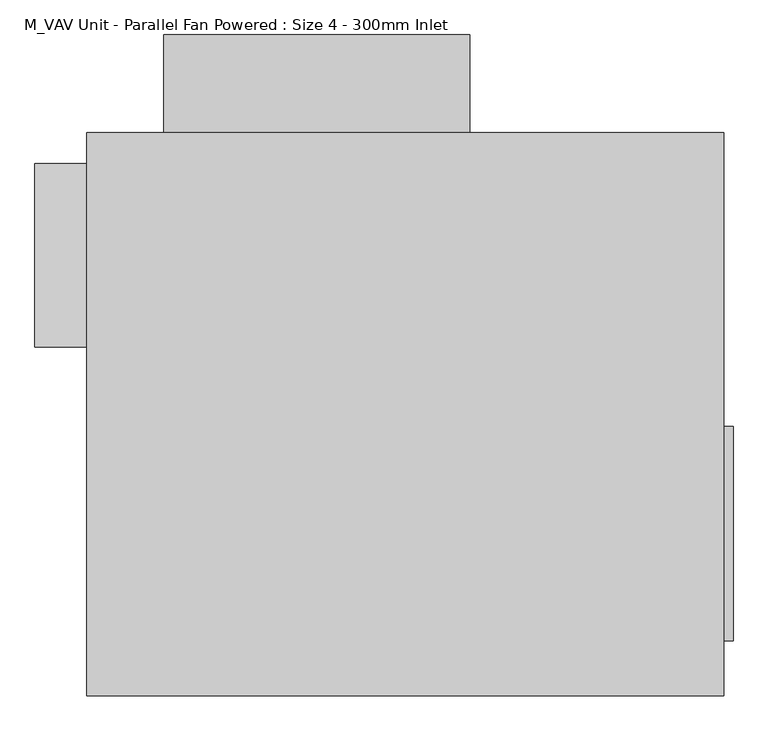
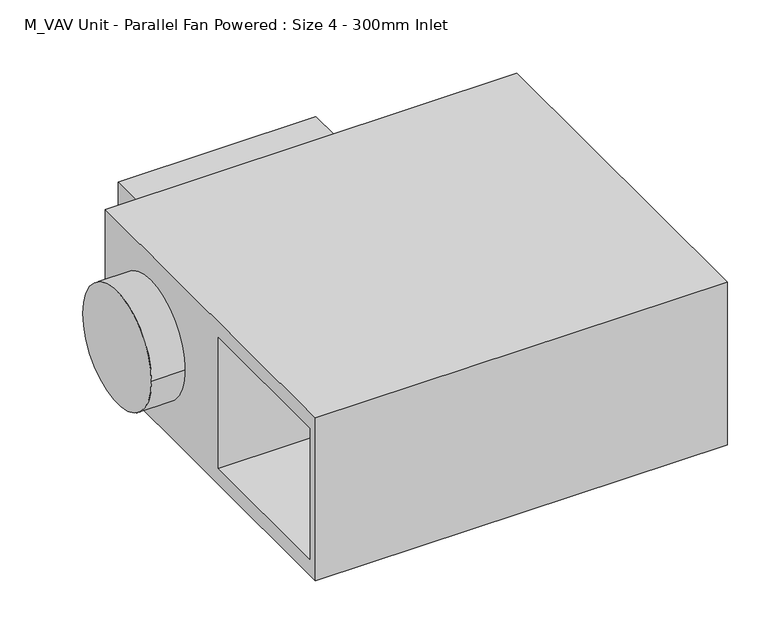
"""IFC4 building model written with IfcOpenShell, lengths in millimetres: proxy geometry, M_VAV Unit - Parallel Fan Powered : Size 4 - 300mm Inlet."""

import ifcopenshell
import ifcopenshell.guid

model = None  # the IFC model being written
_history = None  # IfcOwnerHistory: only IFC2X3 demands one
_inside = {}  # id of a spatial element -> (the spatial element, [elements in it])
_under = {}  # id of a project, library or spatial element -> (it, [spatial elements below it])
_declared = {}  # id of a project -> (the project, [libraries it declares])
_typed = {}  # id of a type object -> (the type object, [elements of that type])
_made_of = {}  # id of a material, layer set ... -> (it, [elements and type objects made of it])


def new_model(schema):
    """Start an empty IFC model of exactly this schema.

    Asked for "IFC4X3", IfcOpenShell would pick the latest addendum, in which some entities
    have other attributes; the version numbers below select the first issue.
    IFC2X3 requires an IfcOwnerHistory on every rooted entity: one is made here for all.
    """
    global model, _history
    if schema == "IFC4X3":
        model = ifcopenshell.file(schema_version=(4, 3, 0, 0))
    else:
        model = ifcopenshell.file(schema=schema)
    _inside.clear()
    _under.clear()
    _declared.clear()
    _typed.clear()
    _made_of.clear()
    _history = None
    if model.schema == "IFC2X3":
        org = make("IfcOrganization", Name="unknown")
        user = make(
            "IfcPersonAndOrganization",
            ThePerson=make("IfcPerson", FamilyName="unknown"),
            TheOrganization=org,
        )
        app = make(
            "IfcApplication",
            ApplicationDeveloper=org,
            Version="unknown",
            ApplicationFullName="unknown",
            ApplicationIdentifier="unknown",
        )
        _history = make(
            "IfcOwnerHistory",
            OwningUser=user,
            OwningApplication=app,
            ChangeAction="ADDED",
            CreationDate=0,
        )
    return model


def make(cls, **values):
    """One entity of the class cls with the attributes given. An attribute that is None is left unset."""
    return model.create_entity(
        cls, **{name: value for name, value in values.items() if value is not None}
    )


def rooted(cls, **values):
    """An entity with a GlobalId (a new one), such as an element, a storey or a relation."""
    return make(cls, GlobalId=ifcopenshell.guid.new(), OwnerHistory=_history, **values)


def si_unit(unit_type, name, prefix=None):
    """IfcSIUnit, for example si_unit("LENGTHUNIT", "METRE", prefix="MILLI")."""
    return make("IfcSIUnit", UnitType=unit_type, Prefix=prefix, Name=name)


def assignment(units):
    """IfcUnitAssignment: the units of a project."""
    return None if units is None else make("IfcUnitAssignment", Units=units)


def point(xyz):
    """IfcCartesianPoint."""
    return None if xyz is None else make("IfcCartesianPoint", Coordinates=xyz)


def direction(xyz):
    """IfcDirection."""
    return None if xyz is None else make("IfcDirection", DirectionRatios=xyz)


def frame(location, z_axis=None, x_axis=None):
    """IfcAxis2Placement3D, a coordinate frame: its origin and axes. An axis left out is left unset."""
    return make(
        "IfcAxis2Placement3D",
        Location=point(location),
        Axis=direction(z_axis),
        RefDirection=direction(x_axis),
    )


def frame_2d(location, x_axis=None):
    """IfcAxis2Placement2D, a coordinate frame in the plane: its origin and x axis."""
    return make(
        "IfcAxis2Placement2D", Location=point(location), RefDirection=direction(x_axis)
    )


def origin():
    """The frame at (0, 0, 0) with its axes left unset."""
    return frame((0.0, 0.0, 0.0))


def place(relative_to, where):
    """IfcLocalPlacement: puts the frame where relative to a parent placement (None: the world)."""
    return make(
        "IfcLocalPlacement", PlacementRelTo=relative_to, RelativePlacement=where
    )


def context(
    kind, dimensions, precision=None, world=None, true_north=None, identifier=None
):
    """IfcGeometricRepresentationContext, for example the 3D "Model" context."""
    return make(
        "IfcGeometricRepresentationContext",
        ContextIdentifier=identifier,
        ContextType=kind,
        CoordinateSpaceDimension=dimensions,
        Precision=precision,
        WorldCoordinateSystem=world,
        TrueNorth=true_north,
    )


def project(units=None, contexts=None):
    """IfcProject with its units and contexts."""
    return rooted(
        "IfcProject",
        Name="project",
        RepresentationContexts=contexts,
        UnitsInContext=assignment(units),
    )


def spatial(cls, under=None, at=None, **own):
    """A site, building, storey or space (cls), placed at a placement, below another one or the project."""
    s = rooted(cls, ObjectPlacement=at, **own)
    if under is not None:
        _under.setdefault(under.id(), (under, []))[1].append(s)
    return s


def polyline(points):
    """IfcPolyline through the points."""
    return make("IfcPolyline", Points=[point(p) for p in points])


def circle_curve(where, radius):
    """IfcCircle in the frame where."""
    return make("IfcCircle", Position=where, Radius=radius)


def trimmed(basis, trim1, trim2, sense, master):
    """IfcTrimmedCurve: the piece of a basis curve between two trims."""
    return make(
        "IfcTrimmedCurve",
        BasisCurve=basis,
        Trim1=trim1,
        Trim2=trim2,
        SenseAgreement=sense,
        MasterRepresentation=master,
    )


def segment(curve, same_sense, transition):
    """IfcCompositeCurveSegment."""
    return make(
        "IfcCompositeCurveSegment",
        Transition=transition,
        SameSense=same_sense,
        ParentCurve=curve,
    )


def composite_curve(segments, self_intersect=None):
    """IfcCompositeCurve: segments joined end to end."""
    return make("IfcCompositeCurve", Segments=segments, SelfIntersect=self_intersect)


def outline(outer, holes=None, kind="AREA"):
    """IfcArbitraryClosedProfileDef: a profile drawn as a closed curve; with holes, ...WithVoids."""
    if holes is None:
        return make("IfcArbitraryClosedProfileDef", ProfileType=kind, OuterCurve=outer)
    return make(
        "IfcArbitraryProfileDefWithVoids",
        ProfileType=kind,
        OuterCurve=outer,
        InnerCurves=holes,
    )


def extrude(swept, where, along, depth):
    """IfcExtrudedAreaSolid: the profile swept, set in the frame where, extruded along a direction by depth."""
    return make(
        "IfcExtrudedAreaSolid",
        SweptArea=swept,
        Position=where,
        ExtrudedDirection=direction(along),
        Depth=depth,
    )


def faces_of(points, faces, orient=None, outer=None):
    """IfcFace entities. A face is a list of loops; a loop is a list of indices into points, from 0.

    orient and outer hold one flag for each loop. By default every Orientation is true, the
    first loop of a face is its IfcFaceOuterBound and the others are IfcFaceBound.
    """
    made = []
    for i, loops in enumerate(faces):
        bounds = []
        for j, loop in enumerate(loops):
            is_outer = j == 0 if outer is None else outer[i][j]
            bounds.append(
                make(
                    "IfcFaceOuterBound" if is_outer else "IfcFaceBound",
                    Bound=make("IfcPolyLoop", Polygon=[points[k] for k in loop]),
                    Orientation=True if orient is None else orient[i][j],
                )
            )
        made.append(make("IfcFace", Bounds=bounds))
    return made


def faceted_brep(points, faces, orient=None, outer=None, voids=None):
    """IfcFacetedBrep: a solid bounded by flat faces; with voids (closed shells), ...WithVoids."""
    shared = [point(p) for p in points]
    hull = make("IfcClosedShell", CfsFaces=faces_of(shared, faces, orient, outer))
    if voids is None:
        return make("IfcFacetedBrep", Outer=hull)
    return make(
        "IfcFacetedBrepWithVoids",
        Outer=hull,
        Voids=[
            make(cls, CfsFaces=faces_of(shared, fs, o, b)) for cls, fs, o, b in voids
        ],
    )


def shape(context_of_items, identifier, shape_type, items):
    """IfcShapeRepresentation: the items that make up one representation, for example the "Body"."""
    return make(
        "IfcShapeRepresentation",
        ContextOfItems=context_of_items,
        RepresentationIdentifier=identifier,
        RepresentationType=shape_type,
        Items=items,
    )


def source(mapping_origin, context_of_items, identifier, shape_type, items):
    """IfcRepresentationMap: a shape defined once, which mapped items show again and again."""
    return make(
        "IfcRepresentationMap",
        MappingOrigin=mapping_origin,
        MappedRepresentation=shape(context_of_items, identifier, shape_type, items),
    )


def transform(
    local_origin,
    x_axis=None,
    y_axis=None,
    z_axis=None,
    scale=None,
    scale2=None,
    scale3=None,
    uniform=True,
):
    """IfcCartesianTransformationOperator3D, or its non-uniform kind. x_axis, y_axis, z_axis: its Axis1, 2, 3."""
    if uniform:
        return make(
            "IfcCartesianTransformationOperator3D",
            Axis1=direction(x_axis),
            Axis2=direction(y_axis),
            LocalOrigin=point(local_origin),
            Scale=scale,
            Axis3=direction(z_axis),
        )
    return make(
        "IfcCartesianTransformationOperator3DnonUniform",
        Axis1=direction(x_axis),
        Axis2=direction(y_axis),
        LocalOrigin=point(local_origin),
        Scale=scale,
        Axis3=direction(z_axis),
        Scale2=scale2,
        Scale3=scale3,
    )


def mapped(mapping_source, mapping_target):
    """IfcMappedItem: shows the shape of a source again, moved by a transform."""
    return make(
        "IfcMappedItem", MappingSource=mapping_source, MappingTarget=mapping_target
    )


def made_of(thing, what):
    """Note that an element or type object is made of a material, layer set ...; save() writes the relation."""
    if what is not None:
        _made_of.setdefault(what.id(), (what, []))[1].append(thing)
    return thing


def element(
    cls,
    number,
    at=None,
    inside=None,
    cuts=None,
    type_object=None,
    material=None,
    context=None,
    identifier="Body",
    shape_type=None,
    held_by="IfcProductDefinitionShape",
    body=None,
    shapes=None,
    **own,
):
    """One element of the class cls, such as IfcWall. Its Tag is "e" and its number.

    at: its placement. inside: the storey or other place that contains it. cuts: it is an
    opening in that element (IfcRelVoidsElement). A single representation is given by context,
    identifier, shape_type and body (its items); several are given by shapes. held_by: the class
    of the entity that holds the representations. save() writes the other relations.
    """
    e = rooted(cls, Tag="e%d" % number, ObjectPlacement=at, **own)
    if body is not None:
        shapes = [shape(context, identifier, shape_type, body)]
    if shapes is not None:
        e.Representation = make(held_by, Representations=shapes)
    if inside is not None:
        _inside.setdefault(inside.id(), (inside, []))[1].append(e)
    if cuts is not None:
        rooted(
            "IfcRelVoidsElement", RelatingBuildingElement=cuts, RelatedOpeningElement=e
        )
    if type_object is not None:
        _typed.setdefault(type_object.id(), (type_object, []))[1].append(e)
    return made_of(e, material)


def aggregate(whole, parts):
    """IfcRelAggregates: a whole, such as a stair, and the parts it consists of."""
    return rooted("IfcRelAggregates", RelatingObject=whole, RelatedObjects=parts)


def save(model, path):
    """Write the relations noted so far, then the file.

    IfcRelAggregates (storeys below a building ...), IfcRelContainedInSpatialStructure (elements
    in a storey), IfcRelDefinesByType, IfcRelAssociatesMaterial and IfcRelDeclares: one each for
    every whole, place, type object, material and project.
    """
    for whole, parts in _under.values():
        aggregate(whole, parts)
    for where, things in _inside.values():
        rooted(
            "IfcRelContainedInSpatialStructure",
            RelatedElements=things,
            RelatingStructure=where,
        )
    for kind, things in _typed.values():
        rooted("IfcRelDefinesByType", RelatedObjects=things, RelatingType=kind)
    for what, things in _made_of.values():
        rooted("IfcRelAssociatesMaterial", RelatedObjects=things, RelatingMaterial=what)
    for by, libraries in _declared.values():
        rooted("IfcRelDeclares", RelatingContext=by, RelatedDefinitions=libraries)
    model.write(path)


def m_vav_unit_parallel_fan_powered_size_4_300mm_inlet_59a1b0b3(model_context):
    return source(origin(), model_context, "Body", "SolidModel", [
        extrude(outline(polyline([(535.0, -20.0), (535.0, -370.0), (519.1125, -370.0), (519.1125, -20.0), (535.0, -20.0)])), frame((0.0, 0.0, -140.0), z_axis=(0.0, 0.0, 1.0), x_axis=(1.0, 0.0, 0.0)), (0.0, 0.0, 1.0), 280.0),
        extrude(outline(polyline([(105.0, 460.0), (-395.0, 460.0), (-395.0, 620.0), (105.0, 620.0), (105.0, 460.0)])), frame((0.0, 0.0, -150.0), z_axis=(0.0, 0.0, 1.0), x_axis=(1.0, 0.0, 0.0)), (0.0, 0.0, 1.0), 300.0),
        extrude(outline(composite_curve([segment(trimmed(circle_curve(frame_2d((260.0, 0.0)), 150.0), [point((110.0, 0.0))], [point((410.0, 0.0))], False, "CARTESIAN"), True, "CONTINUOUS"), segment(trimmed(circle_curve(frame_2d((260.0, 0.0)), 150.0), [point((410.0, 0.0))], [point((110.0, 0.0))], False, "CARTESIAN"), True, "CONTINUOUS")], self_intersect=False)), frame((-605.0, 0.0, 0.0), z_axis=(1.0, 0.0, 0.0), x_axis=(0.0, 1.0, 0.0)), (0.0, 0.0, 1.0), 85.0),
        faceted_brep([(520.0, 460.0, 217.5), (-520.0, 460.0, 217.5), (-520.0, -460.0, 217.5), (520.0, -460.0, 217.5), (520.0, 460.0, -217.5), (520.0, -460.0, -217.5), (-520.0, -460.0, -217.5), (-520.0, 460.0, -217.5), (-520.0, -435.0, 175.0), (-520.0, -435.0, -175.0), (-520.0, -35.0, -175.0), (-520.0, -35.0, 175.0), (0.0, -435.0, 175.0), (0.0, -35.0, 175.0), (0.0, -35.0, -175.0), (0.0, -435.0, -175.0)], [[[0, 1, 2, 3]], [[4, 5, 6, 7]], [[1, 0, 4, 7]], [[2, 1, 7, 6], [8, 9, 10, 11]], [[3, 2, 6, 5]], [[0, 3, 5, 4]], [[12, 13, 14, 15]], [[12, 15, 9, 8]], [[15, 14, 10, 9]], [[14, 13, 11, 10]], [[13, 12, 8, 11]]]),
    ])


if __name__ == "__main__":
    model = new_model("IFC4")
    model_context = context("Model", 3, world=origin())
    ifc_project = project(units=[si_unit("LENGTHUNIT", "METRE", prefix="MILLI")], contexts=[model_context])
    site = spatial("IfcSite", under=ifc_project)
    building = spatial("IfcBuilding", under=site)
    placement = place(None, origin())
    m_vav_unit_parallel_fan_powered_size_4_300mm_inlet_shape = m_vav_unit_parallel_fan_powered_size_4_300mm_inlet_59a1b0b3(model_context)
    element("IfcBuildingElementProxy", 1, Name="M_VAV Unit - Parallel Fan Powered : Size 4 - 300mm Inlet", ObjectType="M_VAV Unit - Parallel Fan Powered : Size 4 - 300mm Inlet", at=placement, inside=building, context=model_context, shape_type="MappedRepresentation", body=[
        mapped(m_vav_unit_parallel_fan_powered_size_4_300mm_inlet_shape, transform((0.0, 0.0, 0.0), x_axis=(1.0, 0.0, 0.0), y_axis=(0.0, 1.0, 0.0), z_axis=(0.0, 0.0, 1.0))),
    ])
    save(model, "model.ifc")

# Revit data of these elements
# Type "M_VAV Unit - Parallel Fan Powered : Size 4 - 300mm Inlet"
#   Model = "45234364"
#   Manufacturer = "Lindab"
#   Description = "VAV box"
#   COBie.Type.CreatedBy = "design@eagle.com"
#   COBie.Type.CreatedOn = "2016-09-13T05:47:35"
#   COBie.Type.Name = "Mechanical Equipment_M_VAV Unit - Parallel Fan Powered_Size 4 - 300mm Inlet"
#   COBie.Type.Category = "23-75 70 21 24 14 : Variable Volume Air Terminal Units"
#   COBie.Type.Description = "VAV box"
#   COBie.Type.Manufacturer = "Lindab"
#   COBie.Type.ModelNumber = "45234364"
#   Model = "45234364"
#   Manufacturer = "Lindab"
#   Description = "VAV box"
#   COBie.Type.ReplacementCost = 0
#   Width2 = 350 mm
#   Voltage = 230 V
#   UnitWidth = 1040 mm
#   UnitHeight = 920 mm
#   UnitDepth = 435 mm
#   SupplyConnectorWidth = 350 mm
#   SupplyConnectorVerticalOffset = 54 mm
#   SupplyConnectorLength = 15 mm
#   SupplyConnectorHorizontalOffset = 90 mm
#   SupplyConnectorDepth = 280 mm
#   SupplyAirConnectorCenterOffset = 265 mm
#   PrimaryToSupplyRatio [instance default] = 0.2
#   PrimaryAirOffset = 200 mm
#   PrimaryAirFlow [instance default] = 188.8 L/s
#   PrimaryAirConnectorVerticalOffset = 217.5 mm
#   PrimaryAirConnectorRadius = 150 mm
#   PrimaryAirConnectorLength = 85 mm
#   PrimaryAirConnectorDiameter = 300 mm
#   PrimaryAirConnectorCenterOffset = 200 mm
#   Pressure Drop [instance default] = 2.5 Pa
#   InducedAirInletWidth = 400 mm
#   InducedAirInletDepth = 350 mm
#   InducedAirConnectorHorizontalOffset = 25 mm
#   InducedAirConnectorCenterOffset = 225 mm
#   Height2 = 280 mm
#   ElectricalConnectionBoxWidth = 500 mm
#   ElectricalConnectionBoxOffset = 125 mm
#   ElectricalConnectionBoxHeight = 160 mm
#   ElectricalConnectionBoxDepth = 300 mm
#   SupplyAirFlow [instance default] = 944.0 L/s
#   Apparent Load = 542 VA
#   COBie.Type = yes
#   SupplyAirConnectorIndex = 2
#   PrimaryAirConnectorIndex = 1
#   Number of Poles = 1
#   InducedAirConnectorIndex = 3
#   VAV Material = none
#   Load Classification = Cooling
#   Assembly Code = ""
# Element 1 (IfcBuildingElementProxy, "M_VAV Unit - Parallel Fan Powered : Size 4 - 300mm Inlet")
#   PrimaryAirFlow = 30.0 L/s
#   SupplyAirFlow = 150.0 L/s
